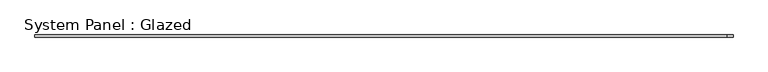
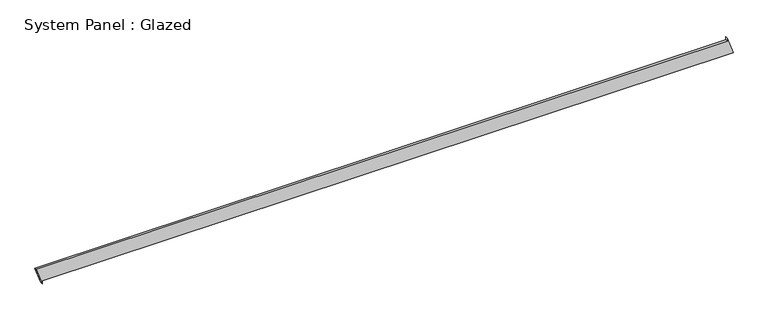
"""IFC4 building model written with IfcOpenShell, lengths in millimetres: plate geometry, System Panel : Glazed."""

from ifc_helpers import new_model, si_unit, frame, origin, place, context, project, spatial, polyline, outline, extrude, source, transform, mapped, element, save


def system_panel_glazed_1607d224(model_context):
    return source(origin(), model_context, "Body", "SweptSolid", [
        extrude(outline(polyline([(0.0, -3958.7518267), (35.3553391, -3958.7518267), (35.3553391, 4028.204431), (235.485295, 3958.8750513), (200.129956, 3958.8752783), (200.0786736, -4028.204431), (0.0, -3958.7518267)])), frame((0.0, -49.5, 0.0), z_axis=(0.0, 1.0, 0.0), x_axis=(0.0, 0.0, 1.0)), (0.0, 0.0, 1.0), 25.0),
    ])


if __name__ == "__main__":
    model = new_model("IFC4")
    model_context = context("Model", 3, world=origin())
    ifc_project = project(units=[si_unit("LENGTHUNIT", "METRE", prefix="MILLI")], contexts=[model_context])
    site = spatial("IfcSite", under=ifc_project)
    building = spatial("IfcBuilding", under=site)
    placement = place(None, origin())
    system_panel_glazed_shape = system_panel_glazed_1607d224(model_context)
    element("IfcPlate", 1, ObjectType="System Panel : Glazed", at=placement, inside=building, context=model_context, shape_type="MappedRepresentation", body=[
        mapped(system_panel_glazed_shape, transform((0.0, 0.0, 0.0), x_axis=(1.0, 0.0, 0.0), y_axis=(0.0, 1.0, 0.0), z_axis=(0.0, 0.0, 1.0))),
    ])
    save(model, "model.ifc")

# Revit data of these elements
# Element 1 (IfcPlate, "System Panel : Glazed")
#   Materials on its faces: "Glass"
# Materials
#   "Glass": class "Glass", colour RGB 218 227 224, transparency 0.85, Description = "Soda Lime Glass", Cost = 0
